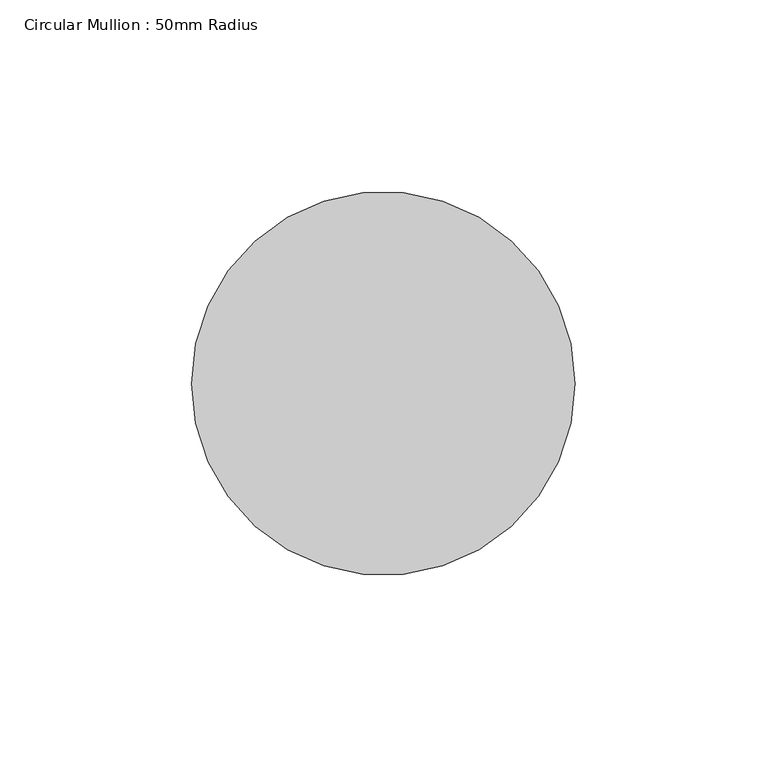
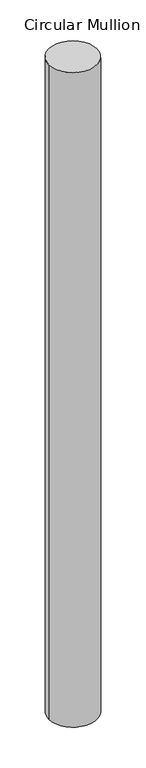
"""IFC4 building model written with IfcOpenShell, lengths in millimetres: member geometry, Circular Mullion : 50mm Radius."""

from ifc_helpers import new_model, si_unit, point, frame, origin, origin_2d, place, context, project, spatial, circle_curve, trimmed, segment, composite_curve, outline, extrude, source, transform, mapped, element, save


def circular_mullion_50mm_radius_72f2cb19(model_context):
    return source(origin(), model_context, "Body", "SweptSolid", [
        extrude(outline(composite_curve([segment(trimmed(circle_curve(origin_2d(), 50.0), [point((50.0, 0.0))], [point((-50.0, 0.0))], False, "CARTESIAN"), True, "CONTINUOUS"), segment(trimmed(circle_curve(origin_2d(), 50.0), [point((-50.0, 0.0))], [point((50.0, 0.0))], False, "CARTESIAN"), True, "CONTINUOUS")], self_intersect=False)), frame((0.0, 0.0, -1439.4819947), z_axis=(0.0, 0.0, 1.0), x_axis=(1.0, 0.0, 0.0)), (0.0, 0.0, 1.0), 1439.4819947),
    ])


if __name__ == "__main__":
    model = new_model("IFC4")
    model_context = context("Model", 3, world=origin())
    ifc_project = project(units=[si_unit("LENGTHUNIT", "METRE", prefix="MILLI")], contexts=[model_context])
    site = spatial("IfcSite", under=ifc_project)
    building = spatial("IfcBuilding", under=site)
    placement = place(None, origin())
    circular_mullion_50mm_radius_shape = circular_mullion_50mm_radius_72f2cb19(model_context)
    element("IfcMember", 1, ObjectType="Circular Mullion : 50mm Radius", at=placement, inside=building, context=model_context, shape_type="MappedRepresentation", body=[
        mapped(circular_mullion_50mm_radius_shape, transform((0.0, 0.0, 0.0), x_axis=(1.0, 0.0, 0.0), y_axis=(0.0, 1.0, 0.0), z_axis=(0.0, 0.0, 1.0))),
    ])
    save(model, "model.ifc")

# Revit data of these elements
# Type "Circular Mullion : 50mm Radius"
#   built-in parameter 1007350 = 0.164042 (stored number, unit not read)
# Element 1 (IfcMember, "Circular Mullion : 50mm Radius")
#   Materials on its faces: "Aluminium"
# Materials
#   "Aluminium": class "Metal", colour RGB 247 247 247, transparency 0, Description = "Aluminium 6061", Cost = 0
